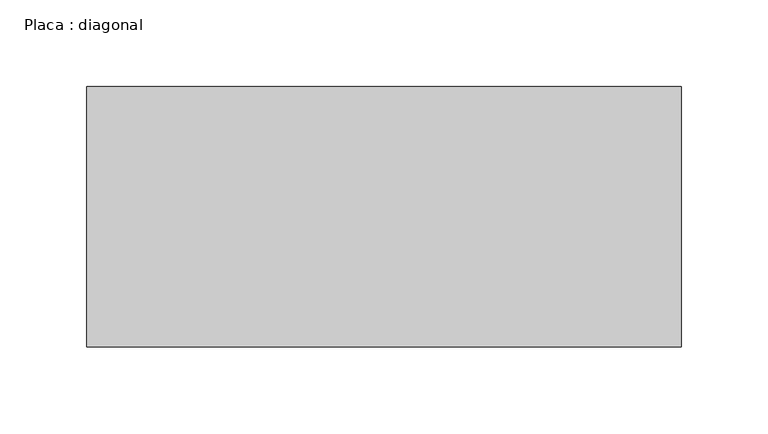
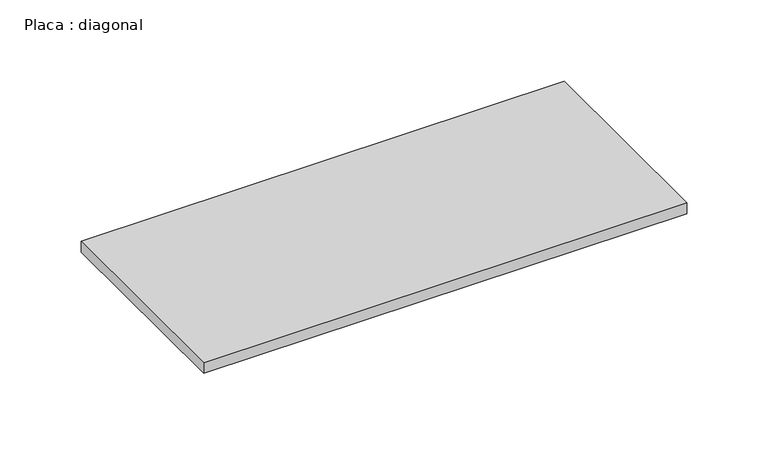
"""IFC4 building model written with IfcOpenShell, lengths in millimetres: beam geometry, Placa : diagonal."""

from ifc_helpers import new_model, si_unit, frame, origin, place, context, project, spatial, polyline, outline, extrude, source, transform, mapped, element, save


def placa_diagonal_54667588(model_context):
    return source(origin(), model_context, "Body", "SweptSolid", [
        extrude(outline(polyline([(170.6977758, 75.0), (170.6977758, -75.0), (-171.6122389, -75.0), (-171.6122389, 75.0), (170.6977758, 75.0)])), frame((0.0, 0.0, -4.0), z_axis=(0.0, 0.0, 1.0), x_axis=(1.0, 0.0, 0.0)), (0.0, 0.0, 1.0), 8.0),
    ])


if __name__ == "__main__":
    model = new_model("IFC4")
    model_context = context("Model", 3, world=origin())
    ifc_project = project(units=[si_unit("LENGTHUNIT", "METRE", prefix="MILLI")], contexts=[model_context])
    site = spatial("IfcSite", under=ifc_project)
    building = spatial("IfcBuilding", under=site)
    placement = place(None, origin())
    placa_diagonal_shape = placa_diagonal_54667588(model_context)
    element("IfcBeam", 1, ObjectType="Placa : diagonal", at=placement, inside=building, context=model_context, shape_type="MappedRepresentation", body=[
        mapped(placa_diagonal_shape, transform((0.0, 0.0, 0.0), x_axis=(1.0, 0.0, 0.0), y_axis=(0.0, 1.0, 0.0), z_axis=(0.0, 0.0, 1.0))),
    ])
    save(model, "model.ifc")

# Revit data of these elements
# Type "Placa : diagonal"
#   W = 0
#   Length [instance default] = 1.50 m
#   b = 0.15 m
#   d = 0.008 m
#   A = 0 m²
#   Structural Material [instance default] = Aço, 45-345
# Element 1 (IfcBeam, "Placa : diagonal")
#   Materials on its faces: "Aço, 45-345"
# Materials
#   "Aço, 45-345": class "Metal", colour RGB 247 247 247, transparency 0, Description = "Aço 345 MPa", Cost = 0
